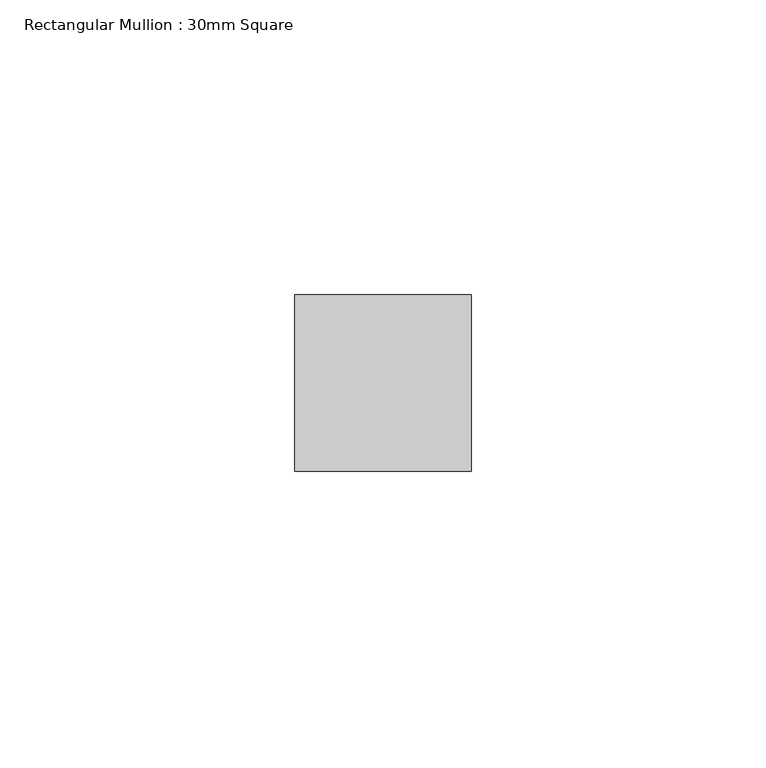
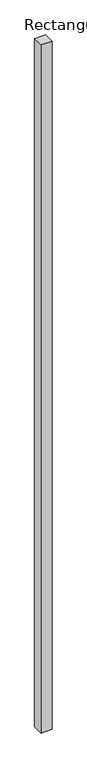
"""IFC4 building model written with IfcOpenShell, lengths in millimetres: member geometry, Rectangular Mullion : 30mm Square."""

from ifc_helpers import new_model, si_unit, frame, origin, place, context, project, spatial, polyline, outline, extrude, source, transform, mapped, element, save


def rectangular_mullion_30mm_square_a7719491(model_context):
    return source(origin(), model_context, "Body", "SweptSolid", [
        extrude(outline(polyline([(15.0, 15.0), (15.0, -15.0), (-15.0, -15.0), (-15.0, 15.0), (15.0, 15.0)])), frame((0.0, 0.0, -1995.0714456), z_axis=(0.0, 0.0, 1.0), x_axis=(1.0, 0.0, 0.0)), (0.0, 0.0, 1.0), 1995.0714456),
    ])


if __name__ == "__main__":
    model = new_model("IFC4")
    model_context = context("Model", 3, world=origin())
    ifc_project = project(units=[si_unit("LENGTHUNIT", "METRE", prefix="MILLI")], contexts=[model_context])
    site = spatial("IfcSite", under=ifc_project)
    building = spatial("IfcBuilding", under=site)
    placement = place(None, origin())
    rectangular_mullion_30mm_square_shape = rectangular_mullion_30mm_square_a7719491(model_context)
    element("IfcMember", 1, ObjectType="Rectangular Mullion : 30mm Square", at=placement, inside=building, context=model_context, shape_type="MappedRepresentation", body=[
        mapped(rectangular_mullion_30mm_square_shape, transform((0.0, 0.0, 0.0), x_axis=(1.0, 0.0, 0.0), y_axis=(0.0, 1.0, 0.0), z_axis=(0.0, 0.0, 1.0))),
    ])
    save(model, "model.ifc")

# Revit data of these elements
# Type "Rectangular Mullion : 30mm Square"
#   built-in parameter 1007304 = 0.0984252 (stored number, unit not read)
#   built-in parameter 1007301 = 0.0492126 (stored number, unit not read)
#   built-in parameter 1007300 = 0.0492126 (stored number, unit not read)
# Element 1 (IfcMember, "Rectangular Mullion : 30mm Square")
#   Materials on its faces: "Aluminum"
# Materials
#   "Aluminum": class "Metal", colour RGB 244 244 244, transparency 0, Description = "Aluminum 6061", Cost = 0
